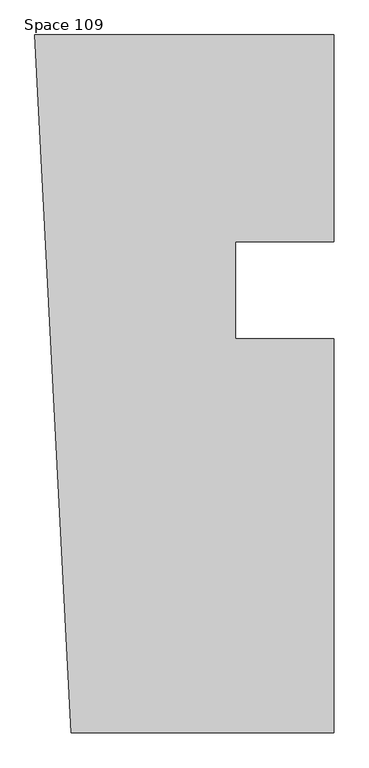
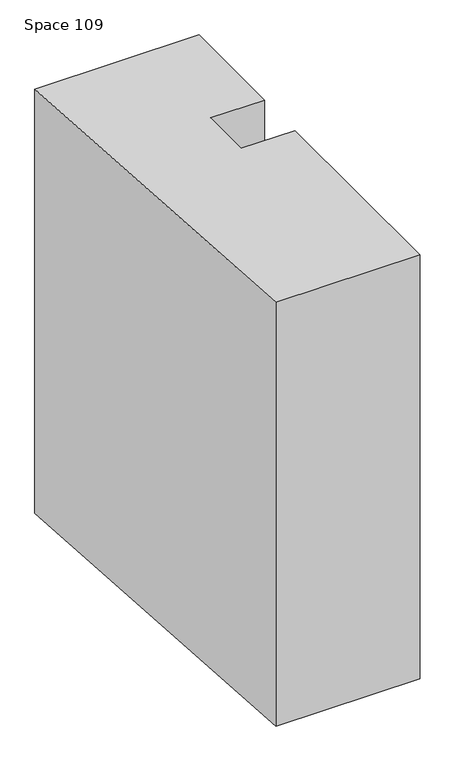
"""IFC4 building model written with IfcOpenShell, lengths in millimetres: proxy geometry, Space 109."""

from ifc_helpers import new_model, si_unit, origin, origin_with_axes, place, context, project, spatial, polyline, outline, extrude, source, transform, mapped, element, save


def space_109_889d3190(model_context):
    return source(origin(), model_context, "Body", "SweptSolid", [
        extrude(outline(polyline([(22026.6059655, 988.215365), (22026.6059655, 626.265365), (22394.9059655, 626.265365), (22394.9059655, -843.759635), (21414.7605841, -843.759635), (21278.3169307, 1759.740365), (22394.9059655, 1759.740365), (22394.9059655, 988.215365), (22026.6059655, 988.215365)])), origin_with_axes(), (0.0, 0.0, 1.0), 3048.0),
    ])


if __name__ == "__main__":
    model = new_model("IFC4")
    model_context = context("Model", 3, world=origin())
    ifc_project = project(units=[si_unit("LENGTHUNIT", "METRE", prefix="MILLI")], contexts=[model_context])
    site = spatial("IfcSite", under=ifc_project)
    building = spatial("IfcBuilding", under=site)
    placement = place(None, origin())
    space_109_shape = space_109_889d3190(model_context)
    element("IfcBuildingElementProxy", 1, Name="Space 109", ObjectType="Space 109", at=placement, inside=building, context=model_context, shape_type="MappedRepresentation", body=[
        mapped(space_109_shape, transform((0.0, 0.0, 0.0), x_axis=(1.0, 0.0, 0.0), y_axis=(0.0, 1.0, 0.0), z_axis=(0.0, 0.0, 1.0))),
    ])
    save(model, "model.ifc")

# Revit data of these elements
# Element 1 (IfcBuildingElementProxy, "Space 109")
#   Materials on its faces: "Render Material 255-255-255"
# Materials
#   "Render Material 255-255-255": class "Unassigned", colour RGB 255 255 255, transparency 0
